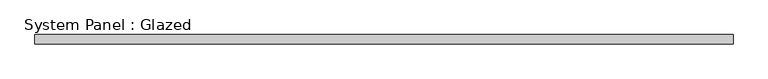
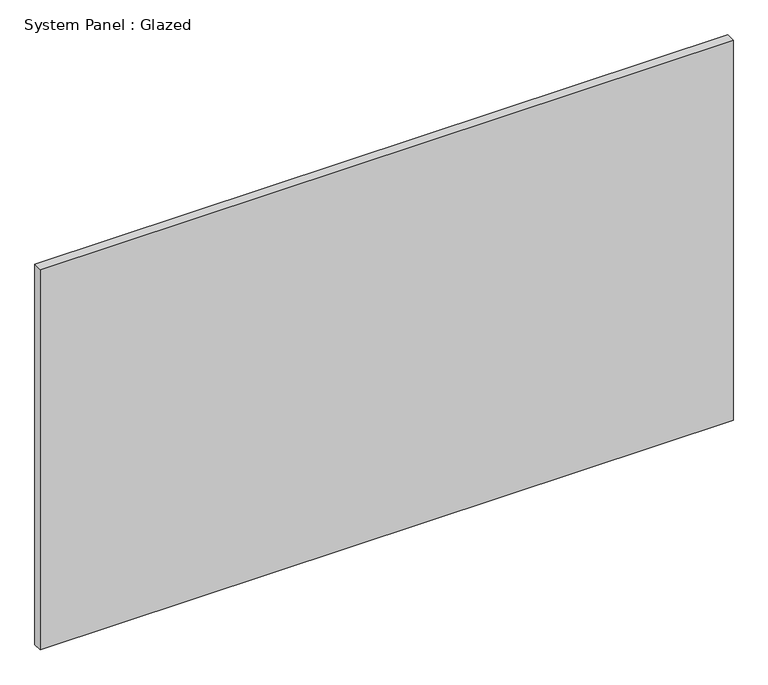
"""IFC4 building model written with IfcOpenShell, lengths in millimetres: plate geometry, System Panel : Glazed."""

from ifc_helpers import new_model, si_unit, origin, origin_with_axes, place, context, project, spatial, polyline, outline, extrude, source, transform, mapped, element, save


def system_panel_glazed_f46199af(model_context):
    return source(origin(), model_context, "Body", "SweptSolid", [
        extrude(outline(polyline([(968.375, -44.45), (-968.375, -44.45), (-968.375, -19.05), (968.375, -19.05), (968.375, -44.45)])), origin_with_axes(), (0.0, 0.0, 1.0), 1123.95),
    ])


if __name__ == "__main__":
    model = new_model("IFC4")
    model_context = context("Model", 3, world=origin())
    ifc_project = project(units=[si_unit("LENGTHUNIT", "METRE", prefix="MILLI")], contexts=[model_context])
    site = spatial("IfcSite", under=ifc_project)
    building = spatial("IfcBuilding", under=site)
    placement = place(None, origin())
    system_panel_glazed_shape = system_panel_glazed_f46199af(model_context)
    element("IfcPlate", 1, ObjectType="System Panel : Glazed", at=placement, inside=building, context=model_context, shape_type="MappedRepresentation", body=[
        mapped(system_panel_glazed_shape, transform((0.0, 0.0, 0.0), x_axis=(1.0, 0.0, 0.0), y_axis=(0.0, 1.0, 0.0), z_axis=(0.0, 0.0, 1.0))),
    ])
    save(model, "model.ifc")

# Revit data of these elements
# Element 1 (IfcPlate, "System Panel : Glazed")
#   Materials on its faces: "Glass"
# Materials
#   "Glass": class "Glass", colour RGB 0 128 192, transparency 0.75
